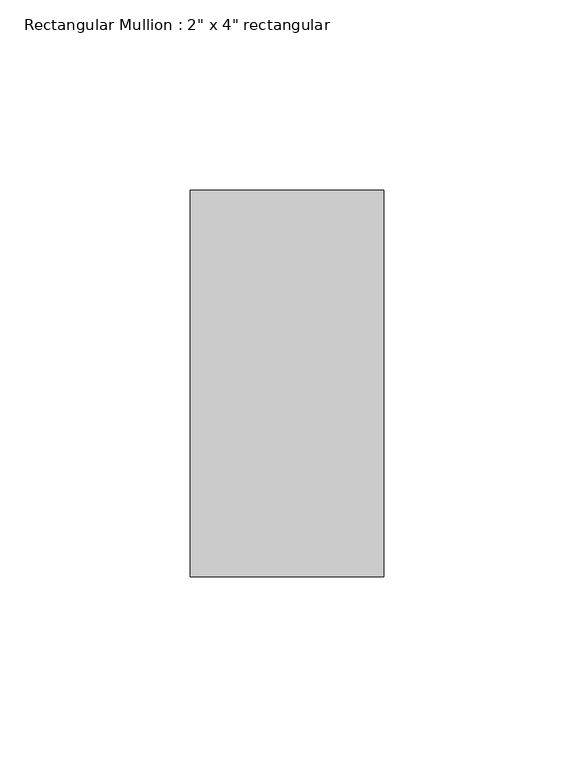
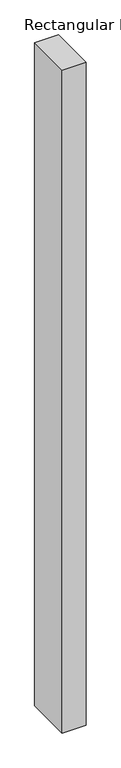
"""IFC4 building model written with IfcOpenShell, lengths in millimetres: member geometry."""

from ifc_helpers import new_model, si_unit, frame, origin, place, context, project, spatial, polyline, outline, extrude, source, transform, mapped, element, save


def member_5c65eda6(model_context):
    return source(origin(), model_context, "Body", "SweptSolid", [
        extrude(outline(polyline([(25.4, 50.8), (25.4, -50.8), (-25.4, -50.8), (-25.4, 50.8), (25.4, 50.8)])), frame((0.0, 0.0, -1493.1571427), z_axis=(0.0, 0.0, 1.0), x_axis=(1.0, 0.0, 0.0)), (0.0, 0.0, 1.0), 1493.1571427),
    ])


if __name__ == "__main__":
    model = new_model("IFC4")
    model_context = context("Model", 3, world=origin())
    ifc_project = project(units=[si_unit("LENGTHUNIT", "METRE", prefix="MILLI")], contexts=[model_context])
    site = spatial("IfcSite", under=ifc_project)
    building = spatial("IfcBuilding", under=site)
    placement = place(None, origin())
    member_shape = member_5c65eda6(model_context)
    element("IfcMember", 1, ObjectType="Rectangular Mullion : 2\" x 4\" rectangular", at=placement, inside=building, context=model_context, shape_type="MappedRepresentation", body=[
        mapped(member_shape, transform((0.0, 0.0, 0.0), x_axis=(1.0, 0.0, 0.0), y_axis=(0.0, 1.0, 0.0), z_axis=(0.0, 0.0, 1.0))),
    ])
    save(model, "model.ifc")

# Revit data of these elements
# Type "Rectangular Mullion : 2\" x 4\" rectangular"
#   built-in parameter 1007304 = 0.333333 (stored number, unit not read)
#   built-in parameter 1007301 = 0.0833333 (stored number, unit not read)
#   built-in parameter 1007300 = 0.0833333 (stored number, unit not read)
